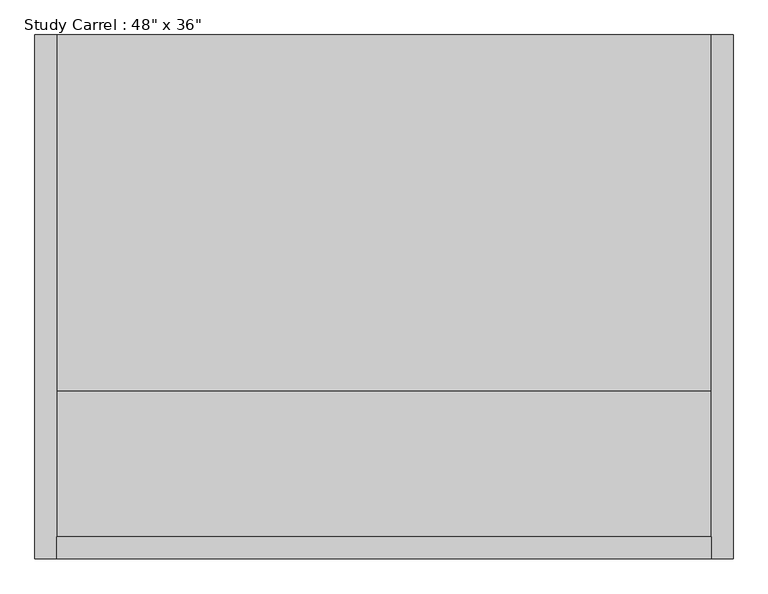
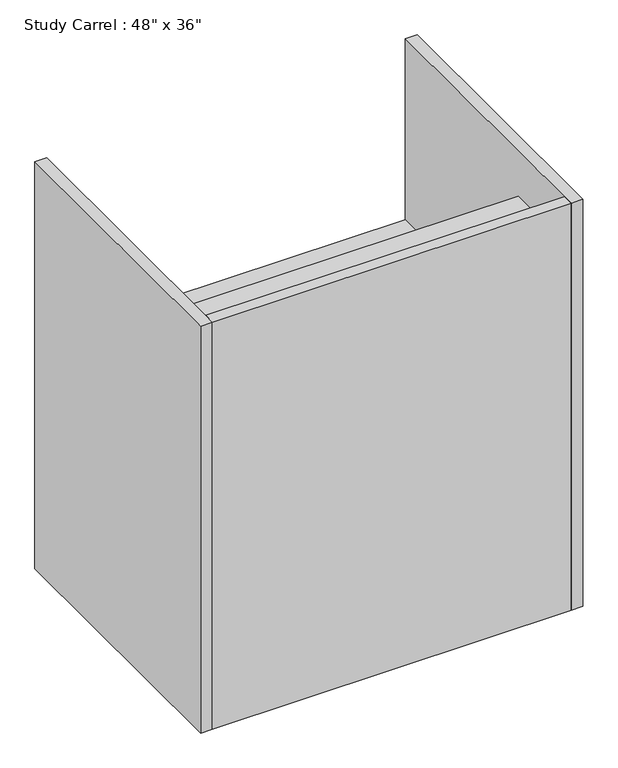
"""IFC4 building model written with IfcOpenShell, lengths in millimetres: furniture geometry."""

from ifc_helpers import new_model, si_unit, frame, origin, origin_with_axes, place, context, project, spatial, polyline, outline, extrude, source, transform, mapped, element, save


def furniture_2f17eec2(model_context):
    return source(origin(), model_context, "Body", "SweptSolid", [
        extrude(outline(polyline([(571.5, -419.1), (-571.5, -419.1), (-571.5, 457.2), (571.5, 457.2), (571.5, -419.1)])), frame((0.0, 0.0, 711.2), z_axis=(0.0, 0.0, 1.0), x_axis=(1.0, 0.0, 0.0)), (0.0, 0.0, 1.0), 50.8),
        extrude(outline(polyline([(571.5, -419.1), (-571.5, -419.1), (-571.5, -165.1), (571.5, -165.1), (571.5, -419.1)])), frame((0.0, 0.0, 1181.1), z_axis=(0.0, 0.0, 1.0), x_axis=(1.0, 0.0, 0.0)), (0.0, 0.0, 1.0), 38.1),
        extrude(outline(polyline([(571.5, -419.1), (571.5, -457.2), (-571.5, -457.2), (-571.5, -419.1), (571.5, -419.1)])), origin_with_axes(), (0.0, 0.0, 1.0), 1371.6),
        extrude(outline(polyline([(609.6, -457.2), (571.5, -457.2), (571.5, 457.2), (609.6, 457.2), (609.6, -457.2)])), origin_with_axes(), (0.0, 0.0, 1.0), 1371.6),
        extrude(outline(polyline([(-571.5, 457.2), (-571.5, -457.2), (-609.6, -457.2), (-609.6, 457.2), (-571.5, 457.2)])), origin_with_axes(), (0.0, 0.0, 1.0), 1371.6),
    ])


if __name__ == "__main__":
    model = new_model("IFC4")
    model_context = context("Model", 3, world=origin())
    ifc_project = project(units=[si_unit("LENGTHUNIT", "METRE", prefix="MILLI")], contexts=[model_context])
    site = spatial("IfcSite", under=ifc_project)
    building = spatial("IfcBuilding", under=site)
    placement = place(None, origin())
    furniture_shape = furniture_2f17eec2(model_context)
    element("IfcFurniture", 1, ObjectType="Study Carrel : 48\" x 36\"", at=placement, inside=building, context=model_context, shape_type="MappedRepresentation", body=[
        mapped(furniture_shape, transform((0.0, 0.0, 0.0), x_axis=(1.0, 0.0, 0.0), y_axis=(0.0, 1.0, 0.0), z_axis=(0.0, 0.0, 1.0))),
    ])
    save(model, "model.ifc")

# Revit data of these elements
# Type "Study Carrel : 48\" x 36\""
#   Assembly Code = "E2020"
#   Depth = 3' - 0"
#   Height = 4' - 6"
#   Width = 4' - 0"
#   Finish = Wood - Birch
#   Default Elevation = 0
# Element 1 (IfcFurniture, "Study Carrel : 48\" x 36\"")
#   Materials on its faces: "Wood - Birch"
# Materials
#   "Wood - Birch": class "Unassigned", colour RGB 224 178 126, transparency 0
